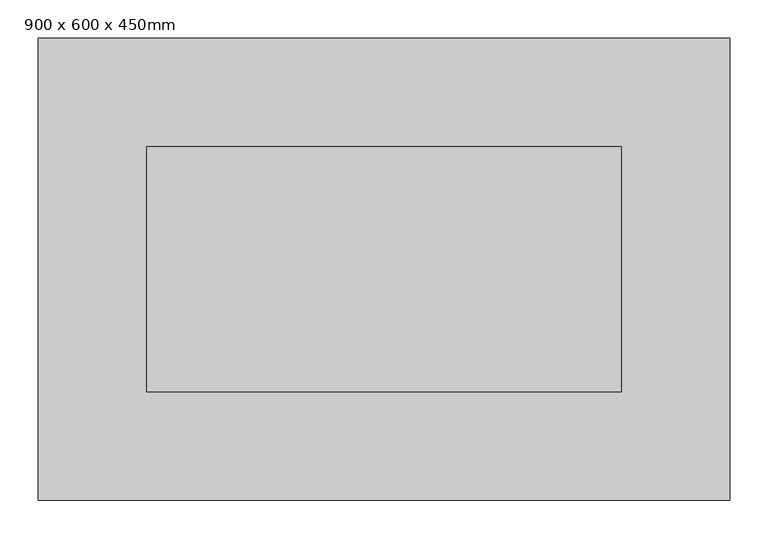
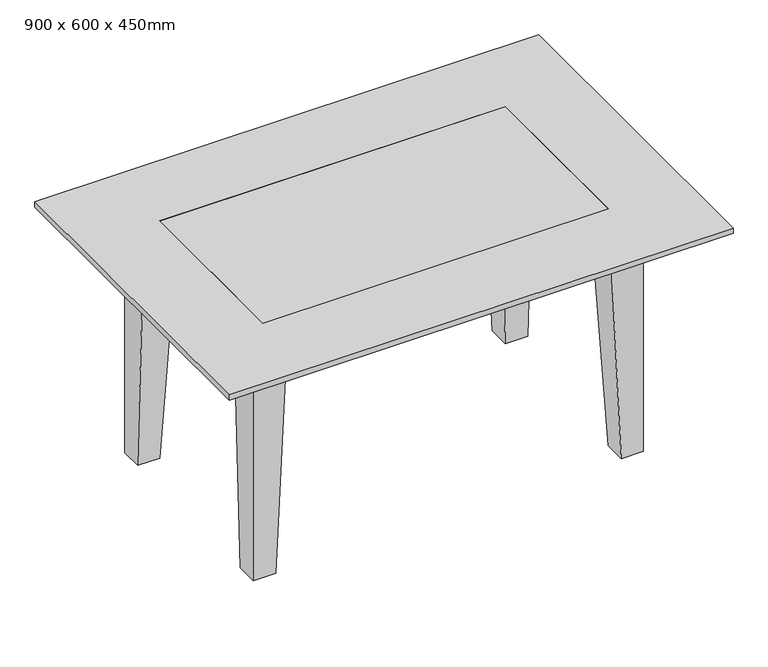
"""IFC4 building model written with IfcOpenShell, lengths in millimetres: furniture geometry, リビングテーブル : 900 x 600 x 450mm."""

from ifc_helpers import new_model, si_unit, frame, origin, place, context, project, spatial, polyline, outline, extrude, faceted_brep, source, transform, mapped, element, save


def furniture_900_x_600_x_450mm_e2215332(model_context):
    return source(origin(), model_context, "Body", "SolidModel", [
        extrude(outline(polyline([(330.0, 180.0), (330.0, -180.0), (-330.0, -180.0), (-330.0, 180.0), (330.0, 180.0)]), holes=[polyline([(290.0, 140.0), (-290.0, 140.0), (-290.0, -140.0), (290.0, -140.0), (290.0, 140.0)])]), frame((0.0, 0.0, 360.0), z_axis=(0.0, 0.0, 1.0), x_axis=(1.0, 0.0, 0.0)), (0.0, 0.0, 1.0), 60.0),
        faceted_brep([(452.0830728, 302.0830728, 440.0), (452.0830728, 302.0830728, 450.0), (452.0830728, -302.0830728, 450.0), (452.0830728, -302.0830728, 440.0), (350.0, 200.0, 420.0), (350.0, -200.0, 420.0), (310.0, 160.0, 450.0), (310.0, 160.0, 420.0), (310.0, -160.0, 420.0), (310.0, -160.0, 450.0), (-452.0830728, -302.0830728, 450.0), (-452.0830728, -302.0830728, 440.0), (-350.0, -200.0, 420.0), (-310.0, -160.0, 420.0), (-310.0, -160.0, 450.0), (-452.0830728, 302.0830728, 450.0), (-452.0830728, 302.0830728, 440.0), (-350.0, 200.0, 420.0), (-310.0, 160.0, 420.0), (-310.0, 160.0, 450.0)], [[[0, 1, 2, 3]], [[4, 0, 3, 5]], [[6, 7, 8, 9]], [[3, 2, 10, 11]], [[5, 3, 11, 12]], [[9, 8, 13, 14]], [[11, 10, 15, 16]], [[12, 11, 16, 17]], [[14, 13, 18, 19]], [[16, 15, 1, 0]], [[17, 16, 0, 4]], [[5, 12, 17, 4], [7, 18, 13, 8]], [[19, 18, 7, 6]], [[1, 15, 10, 2], [9, 14, 19, 6]]]),
        extrude(outline(polyline([(310.0, 160.0), (310.0, -160.0), (-310.0, -160.0), (-310.0, 160.0), (310.0, 160.0)])), frame((0.0, 0.0, 420.0), z_axis=(0.0, 0.0, 1.0), x_axis=(1.0, 0.0, 0.0)), (0.0, 0.0, 1.0), 30.0),
        faceted_brep([(-290.0, -200.0, 420.0), (-290.0, -139.9690818, 420.0), (-350.0, -139.9690818, 420.0), (-350.0, -200.0, 420.0), (-310.0, -200.0, 0.0), (-350.0, -200.0, 0.0), (-350.0, -160.0, 0.0), (-310.0, -160.0, 0.0)], [[[0, 1, 2, 3]], [[4, 5, 6, 7]], [[1, 0, 4, 7]], [[2, 1, 7, 6]], [[3, 2, 6, 5]], [[0, 3, 5, 4]]]),
        faceted_brep([(-290.0, 200.0, 420.0), (-350.0, 200.0, 420.0), (-350.0, 139.9690818, 420.0), (-290.0, 139.9690818, 420.0), (-310.0, 200.0, 0.0), (-310.0, 160.0, 0.0), (-350.0, 160.0, 0.0), (-350.0, 200.0, 0.0)], [[[0, 1, 2, 3]], [[4, 5, 6, 7]], [[1, 0, 4, 7]], [[2, 1, 7, 6]], [[3, 2, 6, 5]], [[0, 3, 5, 4]]]),
        faceted_brep([(290.0, -200.0, 420.0), (350.0, -200.0, 420.0), (350.0, -139.9690818, 420.0), (290.0, -139.9690818, 420.0), (310.0, -200.0, 0.0), (310.0, -160.0, 0.0), (350.0, -160.0, 0.0), (350.0, -200.0, 0.0)], [[[0, 1, 2, 3]], [[4, 5, 6, 7]], [[1, 0, 4, 7]], [[2, 1, 7, 6]], [[3, 2, 6, 5]], [[0, 3, 5, 4]]]),
        faceted_brep([(290.0, 200.0, 420.0), (290.0, 139.9690818, 420.0), (350.0, 139.9690818, 420.0), (350.0, 200.0, 420.0), (310.0, 200.0, 0.0), (350.0, 200.0, 0.0), (350.0, 160.0, 0.0), (310.0, 160.0, 0.0)], [[[0, 1, 2, 3]], [[4, 5, 6, 7]], [[1, 0, 4, 7]], [[2, 1, 7, 6]], [[3, 2, 6, 5]], [[0, 3, 5, 4]]]),
    ])


if __name__ == "__main__":
    model = new_model("IFC4")
    model_context = context("Model", 3, world=origin())
    ifc_project = project(units=[si_unit("LENGTHUNIT", "METRE", prefix="MILLI")], contexts=[model_context])
    site = spatial("IfcSite", under=ifc_project)
    building = spatial("IfcBuilding", under=site)
    placement = place(None, origin())
    furniture_900_x_600_x_450mm_shape = furniture_900_x_600_x_450mm_e2215332(model_context)
    element("IfcFurniture", 1, ObjectType="リビングテーブル : 900 x 600 x 450mm", at=placement, inside=building, context=model_context, shape_type="MappedRepresentation", body=[
        mapped(furniture_900_x_600_x_450mm_shape, transform((0.0, 0.0, 0.0), x_axis=(1.0, 0.0, 0.0), y_axis=(0.0, 1.0, 0.0), z_axis=(0.0, 0.0, 1.0))),
    ])
    save(model, "model.ifc")

# Revit data of these elements
# Type "リビングテーブル : 900 x 600 x 450mm"
#   Keynote = "12490.HH1"
#   高さ = 450 mm
#   幅 = 900 mm
#   奥行き = 600 mm
#   本体 = 木目 - ナチュラル
#   天板内側 = 木目 - ミディアムブラウン
#   Default Elevation = 0
# Element 1 (IfcFurniture, "リビングテーブル : 900 x 600 x 450mm")
#   Materials on its faces: "木目 - ナチュラル", "木目 - ミディアムブラウン"
# Materials
#   "木目 - ナチュラル": class "木材", colour RGB 204 173 122, transparency 0, Cost = 0
#   "木目 - ミディアムブラウン": class "木材", colour RGB 102 44 16, transparency 0, Cost = 0
